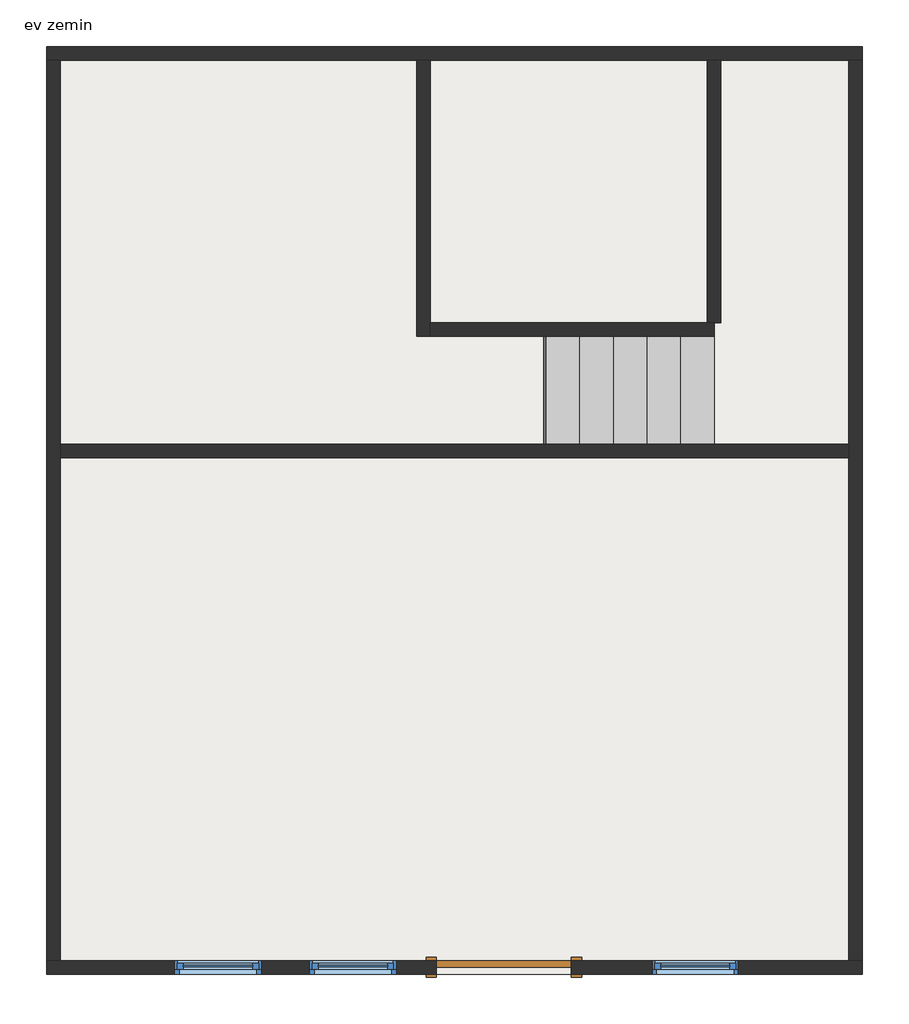
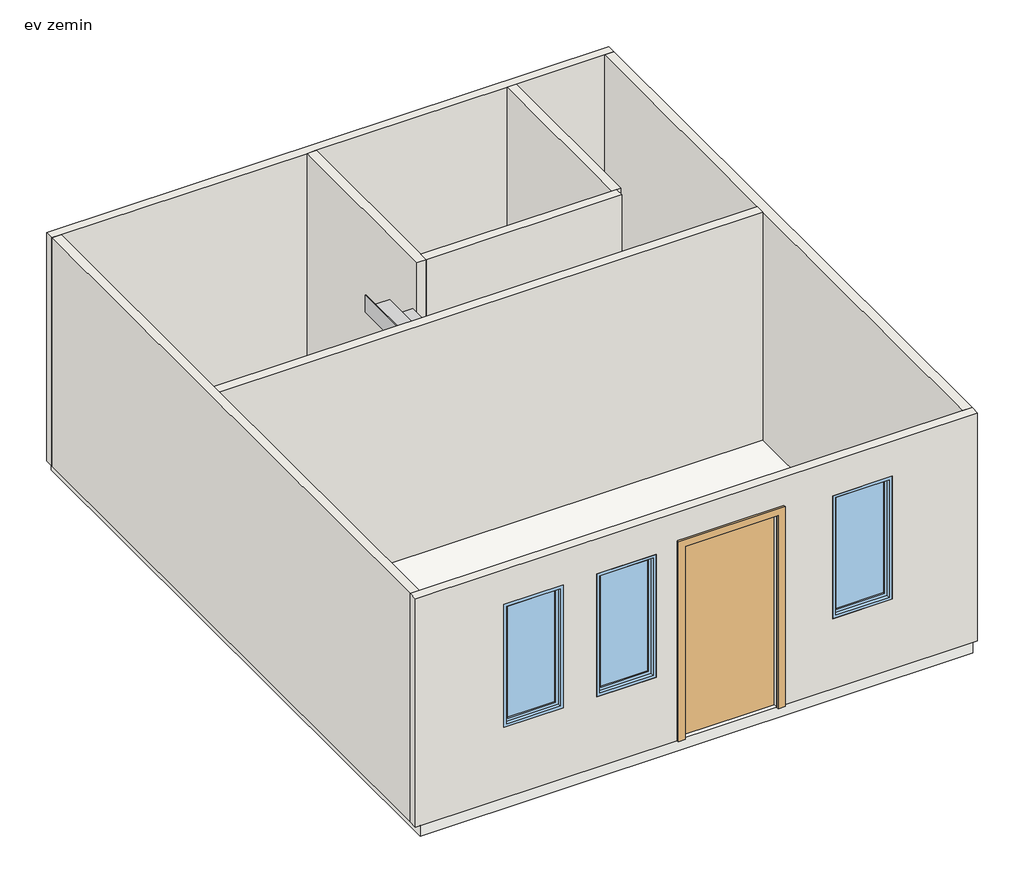
# One storey: 8 walls, 3 windows, 1 door, 1 slab, 1 stair flight.
"""IFC4 building model written with IfcOpenShell, lengths in millimetres."""

import ifcopenshell
import ifcopenshell.guid

model = None  # the IFC model being written
_history = None  # IfcOwnerHistory: only IFC2X3 demands one
_inside = {}  # id of a spatial element -> (the spatial element, [elements in it])
_under = {}  # id of a project, library or spatial element -> (it, [spatial elements below it])
_declared = {}  # id of a project -> (the project, [libraries it declares])
_typed = {}  # id of a type object -> (the type object, [elements of that type])
_made_of = {}  # id of a material, layer set ... -> (it, [elements and type objects made of it])


def new_model(schema):
    """Start an empty IFC model of exactly this schema.

    Asked for "IFC4X3", IfcOpenShell would pick the latest addendum, in which some entities
    have other attributes; the version numbers below select the first issue.
    IFC2X3 requires an IfcOwnerHistory on every rooted entity: one is made here for all.
    """
    global model, _history
    if schema == "IFC4X3":
        model = ifcopenshell.file(schema_version=(4, 3, 0, 0))
    else:
        model = ifcopenshell.file(schema=schema)
    _inside.clear()
    _under.clear()
    _declared.clear()
    _typed.clear()
    _made_of.clear()
    _history = None
    if model.schema == "IFC2X3":
        org = make("IfcOrganization", Name="unknown")
        user = make(
            "IfcPersonAndOrganization",
            ThePerson=make("IfcPerson", FamilyName="unknown"),
            TheOrganization=org,
        )
        app = make(
            "IfcApplication",
            ApplicationDeveloper=org,
            Version="unknown",
            ApplicationFullName="unknown",
            ApplicationIdentifier="unknown",
        )
        _history = make(
            "IfcOwnerHistory",
            OwningUser=user,
            OwningApplication=app,
            ChangeAction="ADDED",
            CreationDate=0,
        )
    return model


def make(cls, **values):
    """One entity of the class cls with the attributes given. An attribute that is None is left unset."""
    return model.create_entity(
        cls, **{name: value for name, value in values.items() if value is not None}
    )


def rooted(cls, **values):
    """An entity with a GlobalId (a new one), such as an element, a storey or a relation."""
    return make(cls, GlobalId=ifcopenshell.guid.new(), OwnerHistory=_history, **values)


def si_unit(unit_type, name, prefix=None):
    """IfcSIUnit, for example si_unit("LENGTHUNIT", "METRE", prefix="MILLI")."""
    return make("IfcSIUnit", UnitType=unit_type, Prefix=prefix, Name=name)


def assignment(units):
    """IfcUnitAssignment: the units of a project."""
    return None if units is None else make("IfcUnitAssignment", Units=units)


def point(xyz):
    """IfcCartesianPoint."""
    return None if xyz is None else make("IfcCartesianPoint", Coordinates=xyz)


def direction(xyz):
    """IfcDirection."""
    return None if xyz is None else make("IfcDirection", DirectionRatios=xyz)


def frame(location, z_axis=None, x_axis=None):
    """IfcAxis2Placement3D, a coordinate frame: its origin and axes. An axis left out is left unset."""
    return make(
        "IfcAxis2Placement3D",
        Location=point(location),
        Axis=direction(z_axis),
        RefDirection=direction(x_axis),
    )


def origin():
    """The frame at (0, 0, 0) with its axes left unset."""
    return frame((0.0, 0.0, 0.0))


def origin_with_axes():
    """The frame at (0, 0, 0) with the z axis (0, 0, 1) and the x axis (1, 0, 0) written out."""
    return frame((0.0, 0.0, 0.0), z_axis=(0.0, 0.0, 1.0), x_axis=(1.0, 0.0, 0.0))


def place(relative_to, where):
    """IfcLocalPlacement: puts the frame where relative to a parent placement (None: the world)."""
    return make(
        "IfcLocalPlacement", PlacementRelTo=relative_to, RelativePlacement=where
    )


def context(
    kind, dimensions, precision=None, world=None, true_north=None, identifier=None
):
    """IfcGeometricRepresentationContext, for example the 3D "Model" context."""
    return make(
        "IfcGeometricRepresentationContext",
        ContextIdentifier=identifier,
        ContextType=kind,
        CoordinateSpaceDimension=dimensions,
        Precision=precision,
        WorldCoordinateSystem=world,
        TrueNorth=true_north,
    )


def project(units=None, contexts=None):
    """IfcProject with its units and contexts."""
    return rooted(
        "IfcProject",
        Name="project",
        RepresentationContexts=contexts,
        UnitsInContext=assignment(units),
    )


def spatial(cls, under=None, at=None, **own):
    """A site, building, storey or space (cls), placed at a placement, below another one or the project."""
    s = rooted(cls, ObjectPlacement=at, **own)
    if under is not None:
        _under.setdefault(under.id(), (under, []))[1].append(s)
    return s


def polyline(points):
    """IfcPolyline through the points."""
    return make("IfcPolyline", Points=[point(p) for p in points])


def outline(outer, holes=None, kind="AREA"):
    """IfcArbitraryClosedProfileDef: a profile drawn as a closed curve; with holes, ...WithVoids."""
    if holes is None:
        return make("IfcArbitraryClosedProfileDef", ProfileType=kind, OuterCurve=outer)
    return make(
        "IfcArbitraryProfileDefWithVoids",
        ProfileType=kind,
        OuterCurve=outer,
        InnerCurves=holes,
    )


def extrude(swept, where, along, depth):
    """IfcExtrudedAreaSolid: the profile swept, set in the frame where, extruded along a direction by depth."""
    return make(
        "IfcExtrudedAreaSolid",
        SweptArea=swept,
        Position=where,
        ExtrudedDirection=direction(along),
        Depth=depth,
    )


def faces_of(points, faces, orient=None, outer=None):
    """IfcFace entities. A face is a list of loops; a loop is a list of indices into points, from 0.

    orient and outer hold one flag for each loop. By default every Orientation is true, the
    first loop of a face is its IfcFaceOuterBound and the others are IfcFaceBound.
    """
    made = []
    for i, loops in enumerate(faces):
        bounds = []
        for j, loop in enumerate(loops):
            is_outer = j == 0 if outer is None else outer[i][j]
            bounds.append(
                make(
                    "IfcFaceOuterBound" if is_outer else "IfcFaceBound",
                    Bound=make("IfcPolyLoop", Polygon=[points[k] for k in loop]),
                    Orientation=True if orient is None else orient[i][j],
                )
            )
        made.append(make("IfcFace", Bounds=bounds))
    return made


def faceted_brep(points, faces, orient=None, outer=None, voids=None):
    """IfcFacetedBrep: a solid bounded by flat faces; with voids (closed shells), ...WithVoids."""
    shared = [point(p) for p in points]
    hull = make("IfcClosedShell", CfsFaces=faces_of(shared, faces, orient, outer))
    if voids is None:
        return make("IfcFacetedBrep", Outer=hull)
    return make(
        "IfcFacetedBrepWithVoids",
        Outer=hull,
        Voids=[
            make(cls, CfsFaces=faces_of(shared, fs, o, b)) for cls, fs, o, b in voids
        ],
    )


def shape(context_of_items, identifier, shape_type, items):
    """IfcShapeRepresentation: the items that make up one representation, for example the "Body"."""
    return make(
        "IfcShapeRepresentation",
        ContextOfItems=context_of_items,
        RepresentationIdentifier=identifier,
        RepresentationType=shape_type,
        Items=items,
    )


def source(mapping_origin, context_of_items, identifier, shape_type, items):
    """IfcRepresentationMap: a shape defined once, which mapped items show again and again."""
    return make(
        "IfcRepresentationMap",
        MappingOrigin=mapping_origin,
        MappedRepresentation=shape(context_of_items, identifier, shape_type, items),
    )


def transform(
    local_origin,
    x_axis=None,
    y_axis=None,
    z_axis=None,
    scale=None,
    scale2=None,
    scale3=None,
    uniform=True,
):
    """IfcCartesianTransformationOperator3D, or its non-uniform kind. x_axis, y_axis, z_axis: its Axis1, 2, 3."""
    if uniform:
        return make(
            "IfcCartesianTransformationOperator3D",
            Axis1=direction(x_axis),
            Axis2=direction(y_axis),
            LocalOrigin=point(local_origin),
            Scale=scale,
            Axis3=direction(z_axis),
        )
    return make(
        "IfcCartesianTransformationOperator3DnonUniform",
        Axis1=direction(x_axis),
        Axis2=direction(y_axis),
        LocalOrigin=point(local_origin),
        Scale=scale,
        Axis3=direction(z_axis),
        Scale2=scale2,
        Scale3=scale3,
    )


def mapped(mapping_source, mapping_target):
    """IfcMappedItem: shows the shape of a source again, moved by a transform."""
    return make(
        "IfcMappedItem", MappingSource=mapping_source, MappingTarget=mapping_target
    )


def made_of(thing, what):
    """Note that an element or type object is made of a material, layer set ...; save() writes the relation."""
    if what is not None:
        _made_of.setdefault(what.id(), (what, []))[1].append(thing)
    return thing


def element(
    cls,
    number,
    at=None,
    inside=None,
    cuts=None,
    type_object=None,
    material=None,
    context=None,
    identifier="Body",
    shape_type=None,
    held_by="IfcProductDefinitionShape",
    body=None,
    shapes=None,
    **own,
):
    """One element of the class cls, such as IfcWall. Its Tag is "e" and its number.

    at: its placement. inside: the storey or other place that contains it. cuts: it is an
    opening in that element (IfcRelVoidsElement). A single representation is given by context,
    identifier, shape_type and body (its items); several are given by shapes. held_by: the class
    of the entity that holds the representations. save() writes the other relations.
    """
    e = rooted(cls, Tag="e%d" % number, ObjectPlacement=at, **own)
    if body is not None:
        shapes = [shape(context, identifier, shape_type, body)]
    if shapes is not None:
        e.Representation = make(held_by, Representations=shapes)
    if inside is not None:
        _inside.setdefault(inside.id(), (inside, []))[1].append(e)
    if cuts is not None:
        rooted(
            "IfcRelVoidsElement", RelatingBuildingElement=cuts, RelatedOpeningElement=e
        )
    if type_object is not None:
        _typed.setdefault(type_object.id(), (type_object, []))[1].append(e)
    return made_of(e, material)


def aggregate(whole, parts):
    """IfcRelAggregates: a whole, such as a stair, and the parts it consists of."""
    return rooted("IfcRelAggregates", RelatingObject=whole, RelatedObjects=parts)


def save(model, path):
    """Write the relations noted so far, then the file.

    IfcRelAggregates (storeys below a building ...), IfcRelContainedInSpatialStructure (elements
    in a storey), IfcRelDefinesByType, IfcRelAssociatesMaterial and IfcRelDeclares: one each for
    every whole, place, type object, material and project.
    """
    for whole, parts in _under.values():
        aggregate(whole, parts)
    for where, things in _inside.values():
        rooted(
            "IfcRelContainedInSpatialStructure",
            RelatedElements=things,
            RelatingStructure=where,
        )
    for kind, things in _typed.values():
        rooted("IfcRelDefinesByType", RelatedObjects=things, RelatingType=kind)
    for what, things in _made_of.values():
        rooted("IfcRelAssociatesMaterial", RelatedObjects=things, RelatingMaterial=what)
    for by, libraries in _declared.values():
        rooted("IfcRelDeclares", RelatingContext=by, RelatedDefinitions=libraries)
    model.write(path)


def m_single_flush_349eedbb(model_context):
    return source(origin(), model_context, "Body", "SweptSolid", [
        extrude(outline(polyline([(2276.0, -576.0), (0.0, -576.0), (0.0, -500.0), (2200.0, -500.0), (2200.0, 500.0), (0.0, 500.0), (0.0, 576.0), (2276.0, 576.0), (2276.0, -576.0)])), frame((0.0, -75.0, 0.0), z_axis=(0.0, 1.0, 0.0), x_axis=(0.0, 0.0, 1.0)), (0.0, 0.0, 1.0), 25.0),
        extrude(outline(polyline([(2276.0, 576.0), (2276.0, -576.0), (0.0, -576.0), (0.0, -500.0), (2200.0, -500.0), (2200.0, 500.0), (0.0, 500.0), (0.0, 576.0), (2276.0, 576.0)])), frame((0.0, 50.0, 0.0), z_axis=(0.0, 1.0, 0.0), x_axis=(0.0, 0.0, 1.0)), (0.0, 0.0, 1.0), 25.0),
        extrude(outline(polyline([(500.0, 1.0), (500.0, -50.0), (-500.0, -50.0), (-500.0, 1.0), (500.0, 1.0)])), origin_with_axes(), (0.0, 0.0, 1.0), 2200.0),
    ])


def stair_flight_50mm_tread_13mm_riser_2ca24aa0(model_context):
    return source(origin(), model_context, "Body", "SweptSolid", [
        extrude(outline(polyline([(-5062.9184352, 4472.0212329), (-5050.4184352, 4472.0212329), (-5050.4184352, 3672.0212329), (-5062.9184352, 3672.0212329), (-5062.9184352, 4472.0212329)])), frame((0.0, 0.0, 200.0), z_axis=(0.0, 0.0, 1.0), x_axis=(1.0, 0.0, 0.0)), (0.0, 0.0, 1.0), 139.3939394),
        extrude(outline(polyline([(-5300.4184352, 3672.0212329), (-5300.4184352, 4472.0212329), (-5050.4184352, 4472.0212329), (-5050.4184352, 3672.0212329), (-5300.4184352, 3672.0212329)])), frame((0.0, 0.0, 339.3939394), z_axis=(0.0, 0.0, 1.0), x_axis=(1.0, 0.0, 0.0)), (0.0, 0.0, 1.0), 50.0),
        extrude(outline(polyline([(-5312.9184352, 4472.0212329), (-5300.4184352, 4472.0212329), (-5300.4184352, 3672.0212329), (-5312.9184352, 3672.0212329), (-5312.9184352, 4472.0212329)])), frame((0.0, 0.0, 339.3939394), z_axis=(0.0, 0.0, 1.0), x_axis=(1.0, 0.0, 0.0)), (0.0, 0.0, 1.0), 189.3939394),
        extrude(outline(polyline([(-5550.4184352, 3672.0212329), (-5550.4184352, 4472.0212329), (-5300.4184352, 4472.0212329), (-5300.4184352, 3672.0212329), (-5550.4184352, 3672.0212329)])), frame((0.0, 0.0, 528.7878788), z_axis=(0.0, 0.0, 1.0), x_axis=(1.0, 0.0, 0.0)), (0.0, 0.0, 1.0), 50.0),
        extrude(outline(polyline([(-5562.9184352, 4472.0212329), (-5550.4184352, 4472.0212329), (-5550.4184352, 3672.0212329), (-5562.9184352, 3672.0212329), (-5562.9184352, 4472.0212329)])), frame((0.0, 0.0, 528.7878788), z_axis=(0.0, 0.0, 1.0), x_axis=(1.0, 0.0, 0.0)), (0.0, 0.0, 1.0), 189.3939394),
        extrude(outline(polyline([(-5800.4184352, 3672.0212329), (-5800.4184352, 4472.0212329), (-5550.4184352, 4472.0212329), (-5550.4184352, 3672.0212329), (-5800.4184352, 3672.0212329)])), frame((0.0, 0.0, 718.1818182), z_axis=(0.0, 0.0, 1.0), x_axis=(1.0, 0.0, 0.0)), (0.0, 0.0, 1.0), 50.0),
        extrude(outline(polyline([(-5812.9184352, 4472.0212329), (-5800.4184352, 4472.0212329), (-5800.4184352, 3672.0212329), (-5812.9184352, 3672.0212329), (-5812.9184352, 4472.0212329)])), frame((0.0, 0.0, 718.1818182), z_axis=(0.0, 0.0, 1.0), x_axis=(1.0, 0.0, 0.0)), (0.0, 0.0, 1.0), 189.3939394),
        extrude(outline(polyline([(-6050.4184352, 3672.0212329), (-6050.4184352, 4472.0212329), (-5800.4184352, 4472.0212329), (-5800.4184352, 3672.0212329), (-6050.4184352, 3672.0212329)])), frame((0.0, 0.0, 907.5757576), z_axis=(0.0, 0.0, 1.0), x_axis=(1.0, 0.0, 0.0)), (0.0, 0.0, 1.0), 50.0),
        extrude(outline(polyline([(-6062.9184352, 4472.0212329), (-6050.4184352, 4472.0212329), (-6050.4184352, 3672.0212329), (-6062.9184352, 3672.0212329), (-6062.9184352, 4472.0212329)])), frame((0.0, 0.0, 907.5757576), z_axis=(0.0, 0.0, 1.0), x_axis=(1.0, 0.0, 0.0)), (0.0, 0.0, 1.0), 189.3939394),
        extrude(outline(polyline([(-6300.4184352, 3672.0212329), (-6300.4184352, 4472.0212329), (-6050.4184352, 4472.0212329), (-6050.4184352, 3672.0212329), (-6300.4184352, 3672.0212329)])), frame((0.0, 0.0, 1096.969697), z_axis=(0.0, 0.0, 1.0), x_axis=(1.0, 0.0, 0.0)), (0.0, 0.0, 1.0), 50.0),
        extrude(outline(polyline([(-6312.9184352, 4472.0212329), (-6300.4184352, 4472.0212329), (-6300.4184352, 3672.0212329), (-6312.9184352, 3672.0212329), (-6312.9184352, 4472.0212329)])), frame((0.0, 0.0, 1096.969697), z_axis=(0.0, 0.0, 1.0), x_axis=(1.0, 0.0, 0.0)), (0.0, 0.0, 1.0), 189.3939394),
        extrude(outline(polyline([(-6550.4184352, 3672.0212329), (-6550.4184352, 4472.0212329), (-6300.4184352, 4472.0212329), (-6300.4184352, 3672.0212329), (-6550.4184352, 3672.0212329)])), frame((0.0, 0.0, 1286.3636364), z_axis=(0.0, 0.0, 1.0), x_axis=(1.0, 0.0, 0.0)), (0.0, 0.0, 1.0), 50.0),
        extrude(outline(polyline([(-6562.9184352, 4472.0212329), (-6550.4184352, 4472.0212329), (-6550.4184352, 3672.0212329), (-6562.9184352, 3672.0212329), (-6562.9184352, 4472.0212329)])), frame((0.0, 0.0, 1286.3636364), z_axis=(0.0, 0.0, 1.0), x_axis=(1.0, 0.0, 0.0)), (0.0, 0.0, 1.0), 189.3939394),
        extrude(outline(polyline([(-6800.4184352, 3672.0212329), (-6800.4184352, 4472.0212329), (-6550.4184352, 4472.0212329), (-6550.4184352, 3672.0212329), (-6800.4184352, 3672.0212329)])), frame((0.0, 0.0, 1475.7575758), z_axis=(0.0, 0.0, 1.0), x_axis=(1.0, 0.0, 0.0)), (0.0, 0.0, 1.0), 50.0),
        extrude(outline(polyline([(-6812.9184352, 4472.0212329), (-6800.4184352, 4472.0212329), (-6800.4184352, 3672.0212329), (-6812.9184352, 3672.0212329), (-6812.9184352, 4472.0212329)])), frame((0.0, 0.0, 1475.7575758), z_axis=(0.0, 0.0, 1.0), x_axis=(1.0, 0.0, 0.0)), (0.0, 0.0, 1.0), 189.3939394),
        extrude(outline(polyline([(-7050.4184352, 3672.0212329), (-7050.4184352, 4472.0212329), (-6800.4184352, 4472.0212329), (-6800.4184352, 3672.0212329), (-7050.4184352, 3672.0212329)])), frame((0.0, 0.0, 1665.1515152), z_axis=(0.0, 0.0, 1.0), x_axis=(1.0, 0.0, 0.0)), (0.0, 0.0, 1.0), 50.0),
        extrude(outline(polyline([(-7062.9184352, 4472.0212329), (-7050.4184352, 4472.0212329), (-7050.4184352, 3672.0212329), (-7062.9184352, 3672.0212329), (-7062.9184352, 4472.0212329)])), frame((0.0, 0.0, 1665.1515152), z_axis=(0.0, 0.0, 1.0), x_axis=(1.0, 0.0, 0.0)), (0.0, 0.0, 1.0), 189.3939394),
        extrude(outline(polyline([(-7300.4184352, 3672.0212329), (-7300.4184352, 4472.0212329), (-7050.4184352, 4472.0212329), (-7050.4184352, 3672.0212329), (-7300.4184352, 3672.0212329)])), frame((0.0, 0.0, 1854.5454545), z_axis=(0.0, 0.0, 1.0), x_axis=(1.0, 0.0, 0.0)), (0.0, 0.0, 1.0), 50.0),
        extrude(outline(polyline([(-7312.9184352, 4472.0212329), (-7300.4184352, 4472.0212329), (-7300.4184352, 3672.0212329), (-7312.9184352, 3672.0212329), (-7312.9184352, 4472.0212329)])), frame((0.0, 0.0, 1854.5454545), z_axis=(0.0, 0.0, 1.0), x_axis=(1.0, 0.0, 0.0)), (0.0, 0.0, 1.0), 189.3939394),
        extrude(outline(polyline([(-7550.4184352, 3672.0212329), (-7550.4184352, 4472.0212329), (-7300.4184352, 4472.0212329), (-7300.4184352, 3672.0212329), (-7550.4184352, 3672.0212329)])), frame((0.0, 0.0, 2043.9393939), z_axis=(0.0, 0.0, 1.0), x_axis=(1.0, 0.0, 0.0)), (0.0, 0.0, 1.0), 50.0),
        extrude(outline(polyline([(-7562.9184352, 4472.0212329), (-7550.4184352, 4472.0212329), (-7550.4184352, 3672.0212329), (-7562.9184352, 3672.0212329), (-7562.9184352, 4472.0212329)])), frame((0.0, 0.0, 2043.9393939), z_axis=(0.0, 0.0, 1.0), x_axis=(1.0, 0.0, 0.0)), (0.0, 0.0, 1.0), 189.3939394),
        extrude(outline(polyline([(-7812.9184352, 4472.0212329), (-7800.4184352, 4472.0212329), (-7800.4184352, 3672.0212329), (-7812.9184352, 3672.0212329), (-7812.9184352, 4472.0212329)])), frame((0.0, 0.0, 2233.3333333), z_axis=(0.0, 0.0, 1.0), x_axis=(1.0, 0.0, 0.0)), (0.0, 0.0, 1.0), 189.3939394),
        extrude(outline(polyline([(-7800.4184352, 3672.0212329), (-7800.4184352, 4472.0212329), (-7550.4184352, 4472.0212329), (-7550.4184352, 3672.0212329), (-7800.4184352, 3672.0212329)])), frame((0.0, 0.0, 2233.3333333), z_axis=(0.0, 0.0, 1.0), x_axis=(1.0, 0.0, 0.0)), (0.0, 0.0, 1.0), 50.0),
    ])


def m_fixed_27182cef(model_context):
    return source(origin(), model_context, "Body", "SweptSolid", [
        extrude(outline(polyline([(-257.0, 28.0), (257.0, 28.0), (257.0, 16.0), (-257.0, 16.0), (-257.0, 28.0)])), frame((0.0, 0.0, 978.0), z_axis=(0.0, 0.0, 1.0), x_axis=(1.0, 0.0, 0.0)), (0.0, 0.0, 1.0), 1274.0),
        extrude(outline(polyline([(2296.0, -301.0), (934.0, -301.0), (934.0, 301.0), (2296.0, 301.0), (2296.0, -301.0)]), holes=[polyline([(2252.0, -257.0), (2252.0, 257.0), (978.0, 257.0), (978.0, -257.0), (2252.0, -257.0)])]), frame((0.0, 0.0, 0.0), z_axis=(0.0, 1.0, 0.0), x_axis=(0.0, 0.0, 1.0)), (0.0, 0.0, 1.0), 44.0),
        extrude(outline(polyline([(2315.0, -320.0), (915.0, -320.0), (915.0, 320.0), (2315.0, 320.0), (2315.0, -320.0)]), holes=[polyline([(2296.0, -301.0), (2296.0, 301.0), (934.0, 301.0), (934.0, -301.0), (2296.0, -301.0)])]), frame((0.0, 0.0, 0.0), z_axis=(0.0, 1.0, 0.0), x_axis=(0.0, 0.0, 1.0)), (0.0, 0.0, 1.0), 63.0),
        extrude(outline(polyline([(2315.0, -320.0), (915.0, -320.0), (915.0, 320.0), (2315.0, 320.0), (2315.0, -320.0)]), holes=[polyline([(2283.0, -288.0), (2283.0, 288.0), (947.0, 288.0), (947.0, -288.0), (2283.0, -288.0)])]), frame((0.0, -37.0, 0.0), z_axis=(0.0, 1.0, 0.0), x_axis=(0.0, 0.0, 1.0)), (0.0, 0.0, 1.0), 37.0),
    ])


model = new_model("IFC4")

# Units and contexts
model_context = context("Model", 3, world=origin())
ifc_project = project(units=[si_unit("LENGTHUNIT", "METRE", prefix="MILLI")], contexts=[model_context])

# Site, building, storey
site = spatial("IfcSite", under=ifc_project)
building = spatial("IfcBuilding", under=site)
storey = spatial("IfcBuildingStorey", under=building, Name="ev zemin", Elevation=0.0)

# Door
placement = place(None, origin())
m_single_flush_shape = m_single_flush_349eedbb(model_context)
element("IfcDoor", 1, ObjectType="M_Single-Flush : 100 x 220 Dış Kapı", at=placement, inside=storey, context=model_context, shape_type="MappedRepresentation", body=[
    mapped(m_single_flush_shape, transform((-6610.4184352, -207.9787671, 0.0), x_axis=(-1.0, 0.0, 0.0), y_axis=(0.0, -1.0, 0.0), z_axis=(0.0, 0.0, 1.0))),
])

# Slab
element("IfcSlab", 2, ObjectType="Concrete- 120 mm", at=placement, inside=storey, context=model_context, shape_type="SweptSolid", body=[
    extrude(outline(polyline([(-4000.4184352, 6622.0212329), (-4000.4184352, -257.9787671), (-9952.5913244, -257.9787671), (-9952.5913244, 6622.0212329), (-4000.4184352, 6622.0212329)])), frame((0.0, 0.0, -120.0), z_axis=(0.0, 0.0, 1.0), x_axis=(1.0, 0.0, 0.0)), (0.0, 0.0, 1.0), 120.0),
])

# Stair flight
stair_flight_50mm_tread_13mm_riser_shape = stair_flight_50mm_tread_13mm_riser_2ca24aa0(model_context)
element("IfcStairFlight", 3, ObjectType="50mm Tread 13mm Riser", at=placement, inside=storey, context=model_context, shape_type="MappedRepresentation", body=[
    mapped(stair_flight_50mm_tread_13mm_riser_shape, transform((0.0, 0.0, 0.0), x_axis=(1.0, 0.0, 0.0), y_axis=(0.0, 1.0, 0.0), z_axis=(0.0, 0.0, 1.0))),
])

# Walls
element("IfcWall", 4, ObjectType="Ahşap 10 cm", at=placement, inside=storey, context=model_context, shape_type="Brep", body=[
    faceted_brep([(-10002.5913244, 6522.0212329, 0.0), (-9902.5913244, 6522.0212329, 0.0), (-7255.4184352, 6522.0212329, 0.0), (-7155.4184352, 6522.0212329, 0.0), (-5100.4184352, 6522.0212329, 0.0), (-5000.4184352, 6522.0212329, 0.0), (-4050.4184352, 6522.0212329, 0.0), (-3950.4184352, 6522.0212329, 0.0), (-3950.4184352, 6522.0212329, 2600.0), (-4050.4184352, 6522.0212329, 2600.0), (-5000.4184352, 6522.0212329, 2600.0), (-5100.4184352, 6522.0212329, 2600.0), (-7155.4184352, 6522.0212329, 2600.0), (-7255.4184352, 6522.0212329, 2600.0), (-9902.5913244, 6522.0212329, 2600.0), (-10002.5913244, 6522.0212329, 2600.0), (-10002.5913244, 6622.0212329, 0.0), (-10002.5913244, 6622.0212329, 2600.0), (-3950.4184352, 6622.0212329, 2600.0), (-3950.4184352, 6622.0212329, 0.0)], [[[0, 1, 2, 3, 4, 5, 6, 7, 8, 9, 10, 11, 12, 13, 14, 15]], [[16, 17, 18, 19]], [[7, 6, 5, 4, 3, 2, 1, 0, 16, 19]], [[15, 14, 13, 12, 11, 10, 9, 8, 18, 17]], [[8, 7, 19, 18]], [[0, 15, 17, 16]]]),
])
element("IfcWall", 5, ObjectType="Ahşap 10 cm", at=placement, inside=storey, context=model_context, shape_type="Brep", body=[
    faceted_brep([(-10002.5913244, -157.9787671, 2600.0), (-9902.5913244, -157.9787671, 2600.0), (-4050.4184352, -157.9787671, 2600.0), (-3950.4184352, -157.9787671, 2600.0), (-3950.4184352, -157.9787671, 0.0), (-4050.4184352, -157.9787671, 0.0), (-6110.4184352, -157.9787671, 0.0), (-6110.4184352, -157.9787671, 2200.0), (-7110.4184352, -157.9787671, 2200.0), (-7110.4184352, -157.9787671, 0.0), (-9902.5913244, -157.9787671, 0.0), (-10002.5913244, -157.9787671, 0.0), (-8410.4184352, -157.9787671, 800.0), (-8410.4184352, -157.9787671, 2200.0), (-9050.4184352, -157.9787671, 2200.0), (-9050.4184352, -157.9787671, 800.0), (-5510.4184352, -157.9787671, 2200.0), (-5510.4184352, -157.9787671, 800.0), (-4870.4184352, -157.9787671, 800.0), (-4870.4184352, -157.9787671, 2200.0), (-8050.4184352, -157.9787671, 2200.0), (-8050.4184352, -157.9787671, 800.0), (-7410.4184352, -157.9787671, 800.0), (-7410.4184352, -157.9787671, 2200.0), (-3950.4184352, -257.9787671, 2600.0), (-10002.5913244, -257.9787671, 2600.0), (-10002.5913244, -257.9787671, 0.0), (-7110.4184352, -257.9787671, 0.0), (-7110.4184352, -257.9787671, 2200.0), (-6110.4184352, -257.9787671, 2200.0), (-6110.4184352, -257.9787671, 0.0), (-3950.4184352, -257.9787671, 0.0), (-8410.4184352, -257.9787671, 2200.0), (-8410.4184352, -257.9787671, 800.0), (-9050.4184352, -257.9787671, 800.0), (-9050.4184352, -257.9787671, 2200.0), (-5510.4184352, -257.9787671, 800.0), (-5510.4184352, -257.9787671, 2200.0), (-4870.4184352, -257.9787671, 2200.0), (-4870.4184352, -257.9787671, 800.0), (-8050.4184352, -257.9787671, 800.0), (-8050.4184352, -257.9787671, 2200.0), (-7410.4184352, -257.9787671, 2200.0), (-7410.4184352, -257.9787671, 800.0)], [[[0, 1, 2, 3, 4, 5, 6, 7, 8, 9, 10, 11], [12, 13, 14, 15], [16, 17, 18, 19], [20, 21, 22, 23]], [[24, 25, 26, 27, 28, 29, 30, 31], [32, 33, 34, 35], [36, 37, 38, 39], [40, 41, 42, 43]], [[27, 26, 11, 10, 9]], [[31, 30, 6, 5, 4]], [[3, 2, 1, 0, 25, 24]], [[12, 33, 32, 13]], [[33, 12, 15, 34]], [[34, 15, 14, 35]], [[13, 32, 35, 14]], [[4, 3, 24, 31]], [[0, 11, 26, 25]], [[9, 8, 28, 27]], [[7, 6, 30, 29]], [[36, 17, 16, 37]], [[38, 19, 18, 39]], [[17, 36, 39, 18]], [[40, 21, 20, 41]], [[22, 43, 42, 23]], [[21, 40, 43, 22]], [[7, 29, 28, 8]], [[19, 38, 37, 16]], [[23, 42, 41, 20]]]),
])
element("IfcWall", 6, ObjectType="Ahşap 10 cm", at=placement, inside=storey, context=model_context, shape_type="SweptSolid", body=[
    extrude(outline(polyline([(-4050.4184352, 3572.0212329), (-9902.5913244, 3572.0212329), (-9902.5913244, 3672.0212329), (-4050.4184352, 3672.0212329), (-4050.4184352, 3572.0212329)])), origin_with_axes(), (0.0, 0.0, 1.0), 2600.0),
])
element("IfcWall", 7, ObjectType="Ahşap 10 cm", at=placement, inside=storey, context=model_context, shape_type="Brep", body=[
    faceted_brep([(-7255.4184352, 6522.0212329, 0.0), (-7255.4184352, 4472.0212329, 0.0), (-7255.4184352, 4472.0212329, 2600.0), (-7255.4184352, 6522.0212329, 2600.0), (-7155.4184352, 6522.0212329, 0.0), (-7155.4184352, 6522.0212329, 2600.0), (-7155.4184352, 4572.0212329, 2600.0), (-7155.4184352, 4472.0212329, 2600.0), (-7155.4184352, 4472.0212329, 0.0), (-7155.4184352, 4572.0212329, 0.0)], [[[0, 1, 2, 3]], [[4, 5, 6, 7, 8, 9]], [[1, 0, 4, 9, 8]], [[3, 2, 7, 6, 5]], [[0, 3, 5, 4]], [[2, 1, 8, 7]]]),
])
element("IfcWall", 8, ObjectType="Ahşap 10 cm", at=placement, inside=storey, context=model_context, shape_type="Brep", body=[
    faceted_brep([(-7155.4184352, 4472.0212329, 0.0), (-5050.4184352, 4472.0212329, 0.0), (-5050.4184352, 4472.0212329, 2600.0), (-7155.4184352, 4472.0212329, 2600.0), (-7155.4184352, 4572.0212329, 0.0), (-7155.4184352, 4572.0212329, 2600.0), (-5100.4184352, 4572.0212329, 2600.0), (-5050.4184352, 4572.0212329, 2600.0), (-5050.4184352, 4572.0212329, 0.0), (-5100.4184352, 4572.0212329, 0.0)], [[[0, 1, 2, 3]], [[4, 5, 6, 7, 8, 9]], [[1, 0, 4, 9, 8]], [[2, 1, 8, 7]], [[3, 2, 7, 6, 5]], [[0, 3, 5, 4]]]),
])
element("IfcWall", 9, ObjectType="Ahşap 10 cm", at=placement, inside=storey, context=model_context, shape_type="Brep", body=[
    faceted_brep([(-5000.4184352, 4572.0212329, 0.0), (-5000.4184352, 6522.0212329, 0.0), (-5000.4184352, 6522.0212329, 2600.0), (-5000.4184352, 4572.0212329, 2600.0), (-5100.4184352, 4572.0212329, 0.0), (-5100.4184352, 4572.0212329, 2600.0), (-5100.4184352, 6522.0212329, 2600.0), (-5100.4184352, 6522.0212329, 0.0), (-5050.4184352, 4572.0212329, 0.0), (-5050.4184352, 4572.0212329, 2600.0)], [[[0, 1, 2, 3]], [[4, 5, 6, 7]], [[1, 0, 8, 4, 7]], [[3, 2, 6, 5, 9]], [[2, 1, 7, 6]], [[0, 3, 9, 5, 4, 8]]]),
])
element("IfcWall", 10, ObjectType="Ahşap 10 cm", at=placement, inside=storey, context=model_context, shape_type="Brep", body=[
    faceted_brep([(-4050.4184352, 6522.0212329, 0.0), (-4050.4184352, 3672.0212329, 0.0), (-4050.4184352, 3572.0212329, 0.0), (-4050.4184352, -157.9787671, 0.0), (-4050.4184352, -157.9787671, 2600.0), (-4050.4184352, 3572.0212329, 2600.0), (-4050.4184352, 3672.0212329, 2600.0), (-4050.4184352, 6522.0212329, 2600.0), (-3950.4184352, 6522.0212329, 0.0), (-3950.4184352, 6522.0212329, 2600.0), (-3950.4184352, -157.9787671, 2600.0), (-3950.4184352, -157.9787671, 0.0)], [[[0, 1, 2, 3, 4, 5, 6, 7]], [[8, 9, 10, 11]], [[3, 2, 1, 0, 8, 11]], [[7, 6, 5, 4, 10, 9]], [[0, 7, 9, 8]], [[4, 3, 11, 10]]]),
])
element("IfcWall", 11, ObjectType="Ahşap 10 cm", at=placement, inside=storey, context=model_context, shape_type="Brep", body=[
    faceted_brep([(-10002.5913244, 6522.0212329, 0.0), (-10002.5913244, -157.9787671, 0.0), (-10002.5913244, -157.9787671, 2600.0), (-10002.5913244, 6522.0212329, 2600.0), (-9902.5913244, 6522.0212329, 0.0), (-9902.5913244, 6522.0212329, 2600.0), (-9902.5913244, 3672.0212329, 2600.0), (-9902.5913244, 3572.0212329, 2600.0), (-9902.5913244, -157.9787671, 2600.0), (-9902.5913244, -157.9787671, 0.0), (-9902.5913244, 3572.0212329, 0.0), (-9902.5913244, 3672.0212329, 0.0)], [[[0, 1, 2, 3]], [[4, 5, 6, 7, 8, 9, 10, 11]], [[1, 0, 4, 11, 10, 9]], [[3, 2, 8, 7, 6, 5]], [[0, 3, 5, 4]], [[2, 1, 9, 8]]]),
])

# Windows
m_fixed_shape = m_fixed_27182cef(model_context)
element("IfcWindow", 12, ObjectType="M_Fixed : 1400 x 640 Ahşap", at=placement, inside=storey, context=model_context, shape_type="MappedRepresentation", body=[
    mapped(m_fixed_shape, transform((-8730.4184352, -220.9787671, -115.0), x_axis=(1.0, 0.0, 0.0), y_axis=(0.0, 1.0, 0.0), z_axis=(0.0, 0.0, 1.0))),
])
element("IfcWindow", 13, ObjectType="M_Fixed : 1400 x 640 Ahşap", at=placement, inside=storey, context=model_context, shape_type="MappedRepresentation", body=[
    mapped(m_fixed_shape, transform((-7730.4184352, -220.9787671, -115.0), x_axis=(1.0, 0.0, 0.0), y_axis=(0.0, 1.0, 0.0), z_axis=(0.0, 0.0, 1.0))),
])
element("IfcWindow", 14, ObjectType="M_Fixed : 1400 x 640 Ahşap", at=placement, inside=storey, context=model_context, shape_type="MappedRepresentation", body=[
    mapped(m_fixed_shape, transform((-5190.4184352, -220.9787671, -115.0), x_axis=(1.0, 0.0, 0.0), y_axis=(0.0, 1.0, 0.0), z_axis=(0.0, 0.0, 1.0))),
])

save(model, "model.ifc")

# Revit data of these elements
# Project information
#   Project Issue Date = "Issue Date"
#   Project Status = "Project Status"
#   Client Name = "Owner"
#   Project Address = "Enter address here"
#   Project Name = "Project Name"
#   Project Number = "0001"
# Type "M_Single-Flush : 100 x 220 Dış Kapı"
#   Type Mark = "23"
#   Construction Type Id = "MDOOR"
#   Analytic Construction = "Metal"
#   Thickness = 5.1 cm
#   Thermal Resistance (R) = 0.270117 (m²·K)/W
#   Heat Transfer Coefficient (U) = 3.7021 W/(m²·K)
#   Height = 220 cm
#   Trim Projection Ext = 2.5 cm
#   Trim Projection Int = 2.5 cm
#   Trim Width = 7.6 cm
#   Width = 100 cm
#   Define Thermal Properties by = 1
#   Door Material = Door - Panel
#   Frame Material = Door - Frame
#   Visual Light Transmittance = 0
#   Solar Heat Gain Coefficient = 0
#   Function = (empty or 0)
#   Wall Closure = (empty or 0)
# Type "Concrete- 120 mm"
#   Function = 0
#   Layers, outside or top first: 11 cm "Concrete, Cast In Situ" (function 1); 0 cm "Damp-proofing" (function 100); 0 cm "Sand" (function 0); 1 cm "Site - Hardcore" (function 0)
# Type "Ahşap 10 cm"
#   Layers, outside or top first: 10 cm no material (function 1)
# Type "M_Fixed : 1400 x 640 Ahşap"
#   Type Mark = "27"
#   Construction Type Id = "GSP4R"
#   Analytic Construction = "1/8 in Pilkington single glazing"
#   Visual Light Transmittance = 0.9
#   Thermal Resistance (R) = 0.271106 (m²·K)/W
#   Solar Heat Gain Coefficient = 0.78
#   Heat Transfer Coefficient (U) = 3.6886 W/(m²·K)
#   Height = 140 cm
#   Default Sill Height = 91.5 cm
#   Width = 64 cm
#   Window Inset = 1.9 cm
#   Define Thermal Properties by = 1
#   Frame Exterior Material = Sash
#   Frame Interior Material = Sash
#   Glass Pane Material = Glass
#   Sash = Sash
#   Wall Closure = (empty or 0)
# Element 1 (IfcDoor, "M_Single-Flush : 100 x 220 Dış Kapı")
#   Phase Created = Phase 1
#   Materials on its faces: "Door - Frame", "Door - Panel"
# Element 2 (IfcSlab, "Concrete- 120 mm")
#   Height Offset From Level = 0 cm
#   Phase Created = Phase 1
#   Materials on its faces: "Site - Hardcore", "Concrete, Cast In Situ"
# Element 3 (IfcStairFlight, "50mm Tread 13mm Riser")
#   Phase Created = Phase 1
# Elements 4, 6, 7, 8 (IfcWall, "Ahşap 10 cm")
#   Top Offset = 0 cm
#   Base Offset = 0 cm
#   Unconnected Height = 260 cm
#   wall height = 260 cm
#   Phase Created = Phase 1
#   Base Constraint = ev zemin
#   Top Constraint = kat 1
#   Materials on its faces: "Default Wall"
# Elements 5, 9, 10, 11 (IfcWall, "Ahşap 10 cm")
#   Top Offset = 0 cm
#   Base Offset = 0 cm
#   wall height = 260 cm
#   Phase Created = Phase 1
#   Base Constraint = ev zemin
#   Top Constraint = kat 1
#   Materials on its faces: "Default Wall"
# Element 12 (IfcWindow, "M_Fixed : 1400 x 640 Ahşap")
#   Mark = "1"
#   Phase Created = Phase 1
#   Materials on its faces: "Sash", "Glass"
# Element 13 (IfcWindow, "M_Fixed : 1400 x 640 Ahşap")
#   Mark = "3"
#   Phase Created = Phase 1
#   Materials on its faces: "Sash", "Glass"
# Element 14 (IfcWindow, "M_Fixed : 1400 x 640 Ahşap")
#   Mark = "5"
#   Phase Created = Phase 1
#   Materials on its faces: "Sash", "Glass"
# Materials
#   "Door - Panel": class "Wood", colour RGB 210 159 95, transparency 0, Cost = 0
#   "Door - Frame": class "Miscellaneous", colour RGB 118 70 51, transparency 0, Cost = 0
#   "Concrete, Cast In Situ": class "Concrete", colour RGB 192 192 192, transparency 0, Description = "physical material", Cost = 0
#   "Damp-proofing": class "Generic", colour RGB 127 127 127, transparency 0, Description = "Damp-proofing", Cost = 0
#   "Sand": class "Generic", colour RGB 191 183 178, transparency 0, Description = "Sand", Cost = 0
#   "Site - Hardcore": class "Miscellaneous", colour RGB 165 42 42, transparency 0, Cost = 0
#   "Sash": class "Wood", colour RGB 224 178 126, transparency 0, Cost = 0
#   "Glass": class "Glass", colour RGB 0 128 192, transparency 0.9, Description = "Soda Lime Glass", Cost = 0
#   "Default Wall": class "Miscellaneous", colour RGB 128 128 128, transparency 0, Cost = 0
